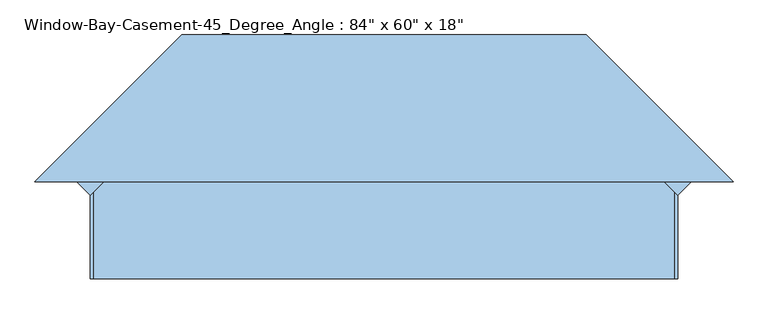
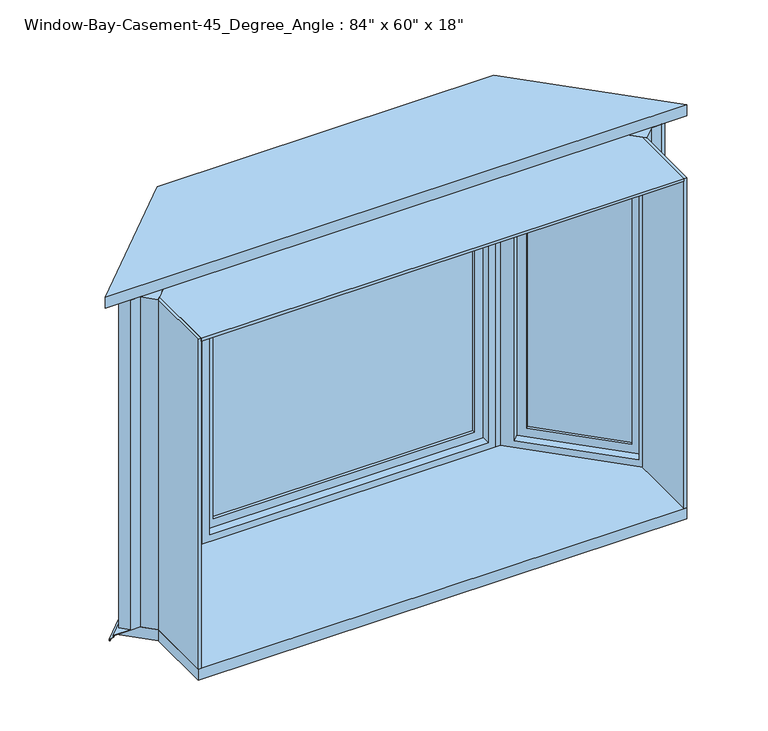
"""IFC4 building model written with IfcOpenShell, lengths in millimetres: window geometry."""

from ifc_helpers import new_model, si_unit, frame, origin, place, context, project, spatial, polyline, outline, extrude, faceted_brep, source, transform, mapped, element, save


def window_84e65bd0(model_context):
    return source(origin(), model_context, "Body", "SolidModel", [
        extrude(outline(polyline([(1066.8, 225.6039087), (1062.3098719, 221.1137806), (771.5637138, 511.8599388), (776.0538418, 516.3500668), (1066.8, 225.6039087)])), frame((0.0, 0.0, 730.25), z_axis=(0.0, 0.0, 1.0), x_axis=(1.0, 0.0, 0.0)), (0.0, 0.0, 1.0), 1384.3),
        extrude(outline(polyline([(1057.8197439, 216.6236525), (1053.3296158, 212.1335245), (762.5834576, 502.8796827), (767.0735857, 507.3698107), (1057.8197439, 216.6236525)])), frame((0.0, 0.0, 730.25), z_axis=(0.0, 0.0, 1.0), x_axis=(1.0, 0.0, 0.0)), (0.0, 0.0, 1.0), 1384.3),
        extrude(outline(polyline([(1441.45, 57.15), (1441.45, -468.3271601), (-57.15, -468.3271601), (-57.15, 57.15), (1441.45, 57.15)]), holes=[polyline([(1384.3, -411.1771601), (1384.3, 0.0), (0.0, 0.0), (0.0, -411.1771601), (1384.3, -411.1771601)])]), frame((1044.3493597, 203.1532684, 730.25), z_axis=(0.7071067811865468, 0.7071067811865483, 0.0), x_axis=(0.0, 0.0, 1.0)), (0.0, 0.0, 1.0), 44.45),
        faceted_brep([(661.8085913, 531.8125, 2184.4), (1066.8, 126.8210913, 2184.4), (1116.1914087, 176.2125, 2184.4), (1161.0926893, 176.2125, 2184.4), (703.8926893, 633.4125, 2184.4), (1084.7605122, 162.7421158, 2171.7), (713.192049, 534.3105791, 2171.7), (758.0933296, 579.2118597, 2171.7), (1129.6617928, 207.6433964, 2171.7), (1044.3493597, 149.2717316, 2152.65), (699.7216648, 493.8994265, 2152.65), (726.6624332, 520.8401949, 2152.65), (1071.2901281, 176.2125, 2152.65), (713.192049, 534.3105791, 673.1), (758.0933296, 579.2118597, 673.1), (699.7216648, 493.8994265, 692.15), (726.6624332, 520.8401949, 692.15), (703.8926893, 633.4125, 660.4), (1161.0926893, 176.2125, 660.4), (1116.1914087, 176.2125, 660.4), (1066.8, 126.8210913, 660.4), (661.8085913, 531.8125, 660.4), (1084.7605122, 162.7421158, 673.1), (1129.6617928, 207.6433964, 673.1), (1044.3493597, 149.2717316, 692.15), (1071.2901281, 176.2125, 692.15)], [[[0, 1, 2, 3, 4]], [[5, 6, 7, 8]], [[9, 10, 11, 12]], [[6, 13, 14, 7]], [[10, 15, 16, 11]], [[17, 18, 19, 20, 21]], [[13, 22, 23, 14]], [[15, 24, 25, 16]], [[20, 19, 2, 1]], [[3, 18, 17, 4], [7, 14, 23, 8]], [[8, 23, 22, 5]], [[5, 22, 13, 6], [11, 16, 25, 12]], [[12, 25, 24, 9]], [[1, 0, 21, 20], [9, 24, 15, 10]], [[4, 17, 21, 0]], [[2, 19, 18, 3]]]),
        extrude(outline(polyline([(-1066.8, 225.6039087), (-776.0538418, 516.3500668), (-771.5637138, 511.8599388), (-1062.3098719, 221.1137806), (-1066.8, 225.6039087)])), frame((0.0, 0.0, 730.25), z_axis=(0.0, 0.0, 1.0), x_axis=(1.0, 0.0, 0.0)), (0.0, 0.0, 1.0), 1384.3),
        extrude(outline(polyline([(-1057.8197439, 216.6236525), (-767.0735857, 507.3698107), (-762.5834576, 502.8796827), (-1053.3296158, 212.1335245), (-1057.8197439, 216.6236525)])), frame((0.0, 0.0, 730.25), z_axis=(0.0, 0.0, 1.0), x_axis=(1.0, 0.0, 0.0)), (0.0, 0.0, 1.0), 1384.3),
        extrude(outline(polyline([(1441.45, -57.15), (-57.15, -57.15), (-57.15, 468.3271601), (1441.45, 468.3271601), (1441.45, -57.15)]), holes=[polyline([(1384.3, 411.1771601), (0.0, 411.1771601), (0.0, 0.0), (1384.3, 0.0), (1384.3, 411.1771601)])]), frame((-1044.3493597, 203.1532684, 730.25), z_axis=(-0.7071067811865468, 0.7071067811865483, 0.0), x_axis=(0.0, 0.0, 1.0)), (0.0, 0.0, 1.0), 44.45),
        faceted_brep([(-661.8085913, 531.8125, 2184.4), (-703.8926893, 633.4125, 2184.4), (-1161.0926893, 176.2125, 2184.4), (-1116.1914087, 176.2125, 2184.4), (-1066.8, 126.8210913, 2184.4), (-1084.7605122, 162.7421158, 2171.7), (-1129.6617928, 207.6433964, 2171.7), (-758.0933296, 579.2118597, 2171.7), (-713.192049, 534.3105791, 2171.7), (-1044.3493597, 149.2717316, 2152.65), (-1071.2901281, 176.2125, 2152.65), (-726.6624332, 520.8401949, 2152.65), (-699.7216648, 493.8994265, 2152.65), (-758.0933296, 579.2118597, 673.1), (-713.192049, 534.3105791, 673.1), (-726.6624332, 520.8401949, 692.15), (-699.7216648, 493.8994265, 692.15), (-703.8926893, 633.4125, 660.4), (-661.8085913, 531.8125, 660.4), (-1066.8, 126.8210913, 660.4), (-1116.1914087, 176.2125, 660.4), (-1161.0926893, 176.2125, 660.4), (-1129.6617928, 207.6433964, 673.1), (-1084.7605122, 162.7421158, 673.1), (-1071.2901281, 176.2125, 692.15), (-1044.3493597, 149.2717316, 692.15)], [[[0, 1, 2, 3, 4]], [[5, 6, 7, 8]], [[9, 10, 11, 12]], [[8, 7, 13, 14]], [[12, 11, 15, 16]], [[17, 18, 19, 20, 21]], [[14, 13, 22, 23]], [[16, 15, 24, 25]], [[19, 4, 3, 20]], [[2, 1, 17, 21], [7, 6, 22, 13]], [[6, 5, 23, 22]], [[5, 8, 14, 23], [11, 10, 24, 15]], [[10, 9, 25, 24]], [[4, 19, 18, 0], [9, 12, 16, 25]], [[1, 0, 18, 17]], [[3, 2, 21, 20]]]),
        faceted_brep([(-724.9347382, 684.2125, 660.4), (-724.9347382, 684.2125, 653.0697935), (724.9347382, 684.2125, 653.0697935), (724.9347382, 684.2125, 660.4), (-703.8926893, 633.4125, 663.1486341), (-703.8926893, 633.4125, 660.4), (703.8926893, 633.4125, 660.4), (703.8926893, 633.4125, 663.1486341), (-725.5133946, 685.6095, 654.4483503), (-725.5133946, 685.6095, 663.1486341), (725.5133946, 685.6095, 663.1486341), (725.5133946, 685.6095, 654.4483503), (730.7739068, 698.3095, 652.2089977), (-730.7739068, 698.3095, 652.2089977), (730.7739068, 698.3095, 643.2668038), (-730.7739068, 698.3095, 643.2668038), (-729.132627, 694.3471, 644.7270038), (-729.132627, 694.3471, 643.2668038), (729.132627, 694.3471, 643.2668038), (729.132627, 694.3471, 644.7270038), (-730.1110823, 696.7093, 650.8662705), (-730.1110823, 696.7093, 644.7270038), (730.1110823, 696.7093, 644.7270038), (730.1110823, 696.7093, 650.8662705), (-1232.9347382, 176.2125, 660.4), (-1232.9347382, 176.2125, 653.0697935), (1232.9347382, 176.2125, 660.4), (1161.0926893, 176.2125, 660.4), (-1161.0926893, 176.2125, 660.4), (-1161.0926893, 176.2125, 663.1486341), (1161.0926893, 176.2125, 663.1486341), (1234.9103945, 176.2125, 663.1486341), (-1234.9103945, 176.2125, 663.1486341), (-1234.9103945, 176.2125, 654.4483503), (-1252.8709068, 176.2125, 652.2089977), (-1252.8709068, 176.2125, 643.2668038), (1252.8709068, 176.2125, 643.2668038), (1247.2672271, 176.2125, 643.2668038), (-1247.2672271, 176.2125, 643.2668038), (-1247.2672271, 176.2125, 644.7270038), (1247.2672271, 176.2125, 644.7270038), (1250.6078823, 176.2125, 644.7270038), (-1250.6078823, 176.2125, 644.7270038), (-1250.6078823, 176.2125, 650.8662705), (1232.9347382, 176.2125, 653.0697935), (1234.9103945, 176.2125, 654.4483503), (1252.8709068, 176.2125, 652.2089977), (1250.6078823, 176.2125, 650.8662705)], [[[0, 1, 2, 3]], [[4, 5, 6, 7]], [[8, 9, 10, 11]], [[8, 11, 12, 13]], [[13, 12, 14, 15]], [[16, 17, 18, 19]], [[20, 21, 22, 23]], [[2, 1, 20, 23]], [[1, 0, 24, 25]], [[0, 3, 26, 27, 6, 5, 28, 24]], [[5, 4, 29, 28]], [[4, 7, 30, 31, 10, 9, 32, 29]], [[9, 8, 33, 32]], [[8, 13, 34, 33]], [[13, 15, 35, 34]], [[15, 14, 36, 37, 18, 17, 38, 35]], [[17, 16, 39, 38]], [[16, 19, 40, 41, 22, 21, 42, 39]], [[21, 20, 43, 42]], [[20, 1, 25, 43]], [[3, 2, 44, 26]], [[7, 6, 27, 30]], [[11, 10, 31, 45]], [[12, 11, 45, 46]], [[14, 12, 46, 36]], [[19, 18, 37, 40]], [[23, 22, 41, 47]], [[2, 23, 47, 44]], [[25, 24, 28, 29, 32, 33, 34, 35, 38, 39, 42, 43]], [[27, 26, 44, 47, 41, 40, 37, 36, 46, 45, 31, 30]]]),
        extrude(outline(polyline([(-1138.642049, 198.6631403), (-1161.0926893, 176.2125), (-1192.5235857, 207.6433964), (-1170.0729454, 230.0940367), (-1138.642049, 198.6631403)])), frame((0.0, 0.0, 663.1486341), z_axis=(0.0, 0.0, 1.0), x_axis=(1.0, 0.0, 0.0)), (0.0, 0.0, 1.0), 1521.2513659),
        extrude(outline(polyline([(1138.642049, 198.6631403), (1170.0729454, 230.0940367), (1192.5235857, 207.6433964), (1161.0926893, 176.2125), (1138.642049, 198.6631403)])), frame((0.0, 0.0, 663.1486341), z_axis=(0.0, 0.0, 1.0), x_axis=(1.0, 0.0, 0.0)), (0.0, 0.0, 1.0), 1521.2513659),
        extrude(outline(polyline([(-661.8085913, 531.8125), (661.8085913, 531.8125), (1054.1, 139.5210913), (1054.1, -176.2125), (-1054.1, -176.2125), (-1054.1, 139.5210913), (-661.8085913, 531.8125)])), frame((0.0, 0.0, 2171.7), z_axis=(0.0, 0.0, 1.0), x_axis=(1.0, 0.0, 0.0)), (0.0, 0.0, 1.0), 12.7),
        extrude(outline(polyline([(-1066.8, -176.2125), (-1066.8, 126.8210913), (-1054.1, 139.5210913), (-1054.1, -176.2125), (-1066.8, -176.2125)])), frame((0.0, 0.0, 660.4), z_axis=(0.0, 0.0, 1.0), x_axis=(1.0, 0.0, 0.0)), (0.0, 0.0, 1.0), 1524.0),
        extrude(outline(polyline([(1066.8, -176.2125), (1054.1, -176.2125), (1054.1, 139.5210913), (1066.8, 126.8210913), (1066.8, -176.2125)])), frame((0.0, 0.0, 660.4), z_axis=(0.0, 0.0, 1.0), x_axis=(1.0, 0.0, 0.0)), (0.0, 0.0, 1.0), 1524.0),
        extrude(outline(polyline([(2171.7, -627.2414087), (673.1, -627.2414087), (673.1, 627.2414087), (2171.7, 627.2414087), (2171.7, -627.2414087)]), holes=[polyline([(2114.55, 570.0914087), (730.25, 570.0914087), (730.25, -570.0914087), (2114.55, -570.0914087), (2114.55, 570.0914087)])]), frame((0.0, 569.9125, 0.0), z_axis=(0.0, 1.0, 0.0), x_axis=(0.0, 0.0, 1.0)), (0.0, 0.0, 1.0), 44.45),
        extrude(outline(polyline([(1066.8, -176.2125), (-1066.8, -176.2125), (-1066.8, 126.8210913), (-1174.5630735, 234.5841648), (-724.9347382, 684.2125), (724.9347382, 684.2125), (1174.5630735, 234.5841648), (1066.8, 126.8210913), (1066.8, -176.2125)])), frame((0.0, 0.0, 609.6), z_axis=(0.0, 0.0, 1.0), x_axis=(1.0, 0.0, 0.0)), (0.0, 0.0, 1.0), 50.8),
        extrude(outline(polyline([(570.0914087, 601.6625), (570.0914087, 595.3125), (-570.0914087, 595.3125), (-570.0914087, 601.6625), (570.0914087, 601.6625)])), frame((0.0, 0.0, 730.25), z_axis=(0.0, 0.0, 1.0), x_axis=(1.0, 0.0, 0.0)), (0.0, 0.0, 1.0), 1384.3),
        extrude(outline(polyline([(570.0914087, 588.9625), (570.0914087, 582.6125), (-570.0914087, 582.6125), (-570.0914087, 588.9625), (570.0914087, 588.9625)])), frame((0.0, 0.0, 730.25), z_axis=(0.0, 0.0, 1.0), x_axis=(1.0, 0.0, 0.0)), (0.0, 0.0, 1.0), 1384.3),
        faceted_brep([(627.2414087, 569.9125, 673.1), (627.2414087, 633.4125, 673.1), (-627.2414087, 633.4125, 673.1), (-627.2414087, 569.9125, 673.1), (608.1914087, 531.8125, 692.15), (608.1914087, 569.9125, 692.15), (-608.1914087, 569.9125, 692.15), (-608.1914087, 531.8125, 692.15), (639.9414087, 633.4125, 660.4), (639.9414087, 531.8125, 660.4), (-639.9414087, 531.8125, 660.4), (-639.9414087, 633.4125, 660.4), (-627.2414087, 633.4125, 2171.7), (-627.2414087, 569.9125, 2171.7), (-608.1914087, 569.9125, 2152.65), (-608.1914087, 531.8125, 2152.65), (-639.9414087, 531.8125, 2184.4), (-639.9414087, 633.4125, 2184.4), (627.2414087, 633.4125, 2171.7), (627.2414087, 569.9125, 2171.7), (608.1914087, 569.9125, 2152.65), (608.1914087, 531.8125, 2152.65), (639.9414087, 531.8125, 2184.4), (639.9414087, 633.4125, 2184.4)], [[[0, 1, 2, 3]], [[4, 5, 6, 7]], [[8, 9, 10, 11]], [[3, 2, 12, 13]], [[7, 6, 14, 15]], [[11, 10, 16, 17]], [[13, 12, 18, 19]], [[15, 14, 20, 21]], [[17, 16, 22, 23]], [[11, 17, 23, 8], [1, 18, 12, 2]], [[19, 18, 1, 0]], [[3, 13, 19, 0], [5, 20, 14, 6]], [[21, 20, 5, 4]], [[9, 22, 16, 10], [7, 15, 21, 4]], [[23, 22, 9, 8]]]),
        extrude(outline(polyline([(-639.9414087, 633.4125), (-639.9414087, 531.8125), (-661.8085913, 531.8125), (-703.8926893, 633.4125), (-639.9414087, 633.4125)])), frame((0.0, 0.0, 660.4), z_axis=(0.0, 0.0, 1.0), x_axis=(1.0, 0.0, 0.0)), (0.0, 0.0, 1.0), 1524.0),
        extrude(outline(polyline([(703.8926893, 633.4125), (661.8085913, 531.8125), (639.9414087, 531.8125), (639.9414087, 633.4125), (703.8926893, 633.4125)])), frame((0.0, 0.0, 660.4), z_axis=(0.0, 0.0, 1.0), x_axis=(1.0, 0.0, 0.0)), (0.0, 0.0, 1.0), 1524.0),
        extrude(outline(polyline([(735.4557627, 709.6125), (1268.8557627, 176.2125), (-1268.8557627, 176.2125), (-735.4557627, 709.6125), (735.4557627, 709.6125)])), frame((0.0, 0.0, 2184.4), z_axis=(0.0, 0.0, 1.0), x_axis=(1.0, 0.0, 0.0)), (0.0, 0.0, 1.0), 50.8),
    ])


if __name__ == "__main__":
    model = new_model("IFC4")
    model_context = context("Model", 3, world=origin())
    ifc_project = project(units=[si_unit("LENGTHUNIT", "METRE", prefix="MILLI")], contexts=[model_context])
    site = spatial("IfcSite", under=ifc_project)
    building = spatial("IfcBuilding", under=site)
    placement = place(None, origin())
    window_shape = window_84e65bd0(model_context)
    element("IfcWindow", 1, ObjectType="Window-Bay-Casement-45_Degree_Angle : 84\" x 60\" x 18\"", at=placement, inside=building, context=model_context, shape_type="MappedRepresentation", body=[
        mapped(window_shape, transform((0.0, 0.0, 0.0), x_axis=(1.0, 0.0, 0.0), y_axis=(0.0, 1.0, 0.0), z_axis=(0.0, 0.0, 1.0))),
    ])
    save(model, "model.ifc")

# Revit data of these elements
# Type "Window-Bay-Casement-45_Degree_Angle : 84\" x 60\" x 18\""
#   Type Mark = "27"
#   Fire Rating = "0.5h"
#   Assembly Code = "B2020100"
#   Analytic Construction = "Double glazing - domestic"
#   Width of Middle Sash = 4' - 2.38909"
#   Width = 7' - 0"
#   Visual Light Transmittance = 0.81
#   Thermal Resistance (R) = 1.8146 (h·ft²·°F)/BTU
#   Solar Heat Gain Coefficient = 0.76
#   Rough Width = 7' - 0 1/2"
#   Rough Height = 5' - 0 1/2"
#   Length 4 = 0' - 1.13909"
#   Length 3 = 0' - 0.51777"
#   Length 2 = 4' - 7.42462"
#   Length 1 = 1' - 2.80546"
#   Wall Thickness [instance default] = 0' - 6"
#   Trim Width = 7' - 5.03553"
#   Trim Height = 5' - 0"
#   Height 1 = 5' - 2"
#   Height = 5' - 0"
#   Heat Transfer Coefficient (U) = 0.5511 BTU/(h·ft²·°F)
#   Depth = 1' - 6"
#   Default Sill Height = 2' - 0"
#   Angle 1 = 22.5000°
#   Angle = 45.0000°
#   Center Muntin Visibility = yes
#   Side Muntin Visibility = yes
#   Interior Trim Visibility [instance default] = yes
#   Exterior Trim Visibility [instance default] = yes
#   Center Muntin Pattern = Muntin Pattern_2x2 : Muntin Pattern_2x2
#   Side Muntin Pattern = Muntin Pattern_2x2 : Muntin Pattern_2x2
#   Interior Trim Material = Wood - Stained
#   Exterior Trim Material = Clad - White
#   Exterior Trim = element 422174
#   Interior Trim = Trim-Window-Interior-Flat : Picture Frame
#   Interior Frame Material = Wood - Stained
#   Glass Panel Material = Glass
#   Exterior Frame Material = Clad - White
#   Wall Closure = (empty or 0)
# Element 1 (IfcWindow, "Window-Bay-Casement-45_Degree_Angle : 84\" x 60\" x 18\"")
#   Wall Thickness = 1' - 1 7/8"
#   Materials on its faces: "Wood - Stained", "Clad - White", "Glass"
# Materials
#   "Wood - Stained": class "Wood", colour RGB 224 178 126, transparency 0, Cost = 0
#   "Clad - White": class "Wood", colour RGB 242 242 238, transparency 0, Cost = 0
#   "Glass": class "Glass", colour RGB 0 128 192, transparency 0.75, Description = "Soda Lime Glass", Cost = 0
